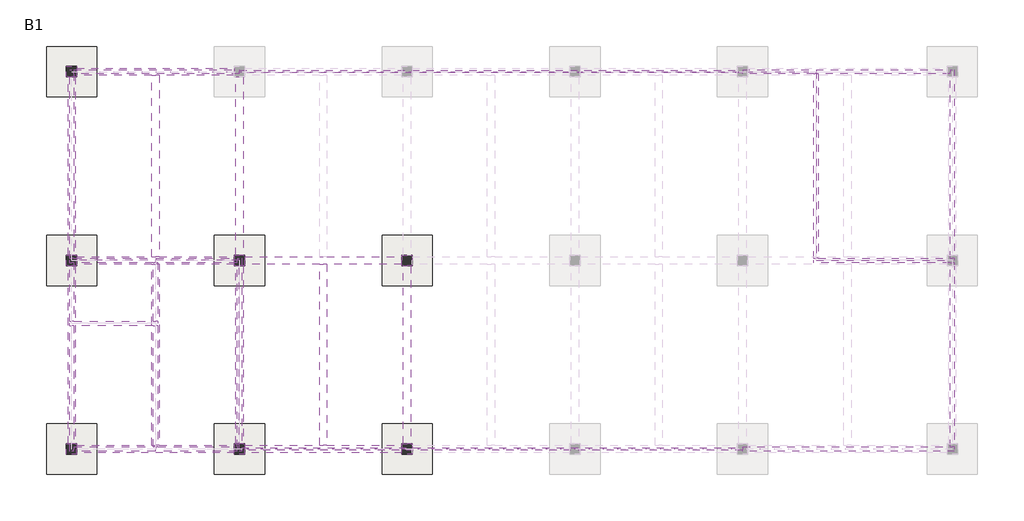
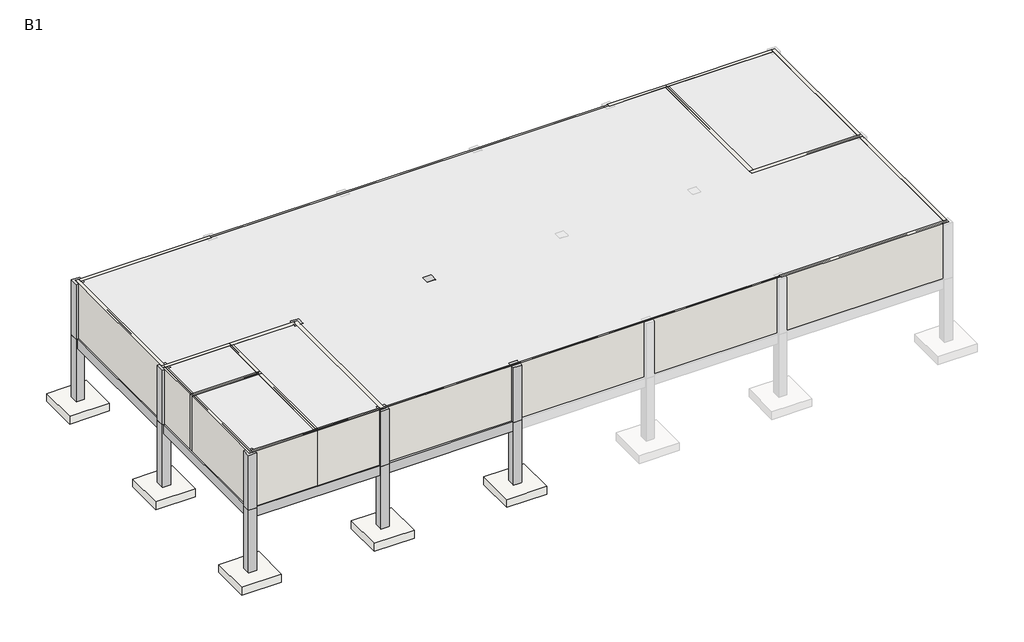
# One storey, part 1 of 2: 21 walls, 14 columns, 13 beams, 12 slabs.
"""IFC4 building model written with IfcOpenShell, lengths in millimetres."""

import ifcopenshell
import ifcopenshell.guid

model = None  # the IFC model being written
_history = None  # IfcOwnerHistory: only IFC2X3 demands one
_inside = {}  # id of a spatial element -> (the spatial element, [elements in it])
_under = {}  # id of a project, library or spatial element -> (it, [spatial elements below it])
_declared = {}  # id of a project -> (the project, [libraries it declares])
_typed = {}  # id of a type object -> (the type object, [elements of that type])
_made_of = {}  # id of a material, layer set ... -> (it, [elements and type objects made of it])


def new_model(schema):
    """Start an empty IFC model of exactly this schema.

    Asked for "IFC4X3", IfcOpenShell would pick the latest addendum, in which some entities
    have other attributes; the version numbers below select the first issue.
    IFC2X3 requires an IfcOwnerHistory on every rooted entity: one is made here for all.
    """
    global model, _history
    if schema == "IFC4X3":
        model = ifcopenshell.file(schema_version=(4, 3, 0, 0))
    else:
        model = ifcopenshell.file(schema=schema)
    _inside.clear()
    _under.clear()
    _declared.clear()
    _typed.clear()
    _made_of.clear()
    _history = None
    if model.schema == "IFC2X3":
        org = make("IfcOrganization", Name="unknown")
        user = make(
            "IfcPersonAndOrganization",
            ThePerson=make("IfcPerson", FamilyName="unknown"),
            TheOrganization=org,
        )
        app = make(
            "IfcApplication",
            ApplicationDeveloper=org,
            Version="unknown",
            ApplicationFullName="unknown",
            ApplicationIdentifier="unknown",
        )
        _history = make(
            "IfcOwnerHistory",
            OwningUser=user,
            OwningApplication=app,
            ChangeAction="ADDED",
            CreationDate=0,
        )
    return model


def make(cls, **values):
    """One entity of the class cls with the attributes given. An attribute that is None is left unset."""
    return model.create_entity(
        cls, **{name: value for name, value in values.items() if value is not None}
    )


def rooted(cls, **values):
    """An entity with a GlobalId (a new one), such as an element, a storey or a relation."""
    return make(cls, GlobalId=ifcopenshell.guid.new(), OwnerHistory=_history, **values)


def si_unit(unit_type, name, prefix=None):
    """IfcSIUnit, for example si_unit("LENGTHUNIT", "METRE", prefix="MILLI")."""
    return make("IfcSIUnit", UnitType=unit_type, Prefix=prefix, Name=name)


def assignment(units):
    """IfcUnitAssignment: the units of a project."""
    return None if units is None else make("IfcUnitAssignment", Units=units)


def point(xyz):
    """IfcCartesianPoint."""
    return None if xyz is None else make("IfcCartesianPoint", Coordinates=xyz)


def direction(xyz):
    """IfcDirection."""
    return None if xyz is None else make("IfcDirection", DirectionRatios=xyz)


def frame(location, z_axis=None, x_axis=None):
    """IfcAxis2Placement3D, a coordinate frame: its origin and axes. An axis left out is left unset."""
    return make(
        "IfcAxis2Placement3D",
        Location=point(location),
        Axis=direction(z_axis),
        RefDirection=direction(x_axis),
    )


def origin():
    """The frame at (0, 0, 0) with its axes left unset."""
    return frame((0.0, 0.0, 0.0))


def origin_with_axes():
    """The frame at (0, 0, 0) with the z axis (0, 0, 1) and the x axis (1, 0, 0) written out."""
    return frame((0.0, 0.0, 0.0), z_axis=(0.0, 0.0, 1.0), x_axis=(1.0, 0.0, 0.0))


def place(relative_to, where):
    """IfcLocalPlacement: puts the frame where relative to a parent placement (None: the world)."""
    return make(
        "IfcLocalPlacement", PlacementRelTo=relative_to, RelativePlacement=where
    )


def context(
    kind, dimensions, precision=None, world=None, true_north=None, identifier=None
):
    """IfcGeometricRepresentationContext, for example the 3D "Model" context."""
    return make(
        "IfcGeometricRepresentationContext",
        ContextIdentifier=identifier,
        ContextType=kind,
        CoordinateSpaceDimension=dimensions,
        Precision=precision,
        WorldCoordinateSystem=world,
        TrueNorth=true_north,
    )


def project(units=None, contexts=None):
    """IfcProject with its units and contexts."""
    return rooted(
        "IfcProject",
        Name="project",
        RepresentationContexts=contexts,
        UnitsInContext=assignment(units),
    )


def spatial(cls, under=None, at=None, **own):
    """A site, building, storey or space (cls), placed at a placement, below another one or the project."""
    s = rooted(cls, ObjectPlacement=at, **own)
    if under is not None:
        _under.setdefault(under.id(), (under, []))[1].append(s)
    return s


def polyline(points):
    """IfcPolyline through the points."""
    return make("IfcPolyline", Points=[point(p) for p in points])


def outline(outer, holes=None, kind="AREA"):
    """IfcArbitraryClosedProfileDef: a profile drawn as a closed curve; with holes, ...WithVoids."""
    if holes is None:
        return make("IfcArbitraryClosedProfileDef", ProfileType=kind, OuterCurve=outer)
    return make(
        "IfcArbitraryProfileDefWithVoids",
        ProfileType=kind,
        OuterCurve=outer,
        InnerCurves=holes,
    )


def extrude(swept, where, along, depth):
    """IfcExtrudedAreaSolid: the profile swept, set in the frame where, extruded along a direction by depth."""
    return make(
        "IfcExtrudedAreaSolid",
        SweptArea=swept,
        Position=where,
        ExtrudedDirection=direction(along),
        Depth=depth,
    )


def faces_of(points, faces, orient=None, outer=None):
    """IfcFace entities. A face is a list of loops; a loop is a list of indices into points, from 0.

    orient and outer hold one flag for each loop. By default every Orientation is true, the
    first loop of a face is its IfcFaceOuterBound and the others are IfcFaceBound.
    """
    made = []
    for i, loops in enumerate(faces):
        bounds = []
        for j, loop in enumerate(loops):
            is_outer = j == 0 if outer is None else outer[i][j]
            bounds.append(
                make(
                    "IfcFaceOuterBound" if is_outer else "IfcFaceBound",
                    Bound=make("IfcPolyLoop", Polygon=[points[k] for k in loop]),
                    Orientation=True if orient is None else orient[i][j],
                )
            )
        made.append(make("IfcFace", Bounds=bounds))
    return made


def faceted_brep(points, faces, orient=None, outer=None, voids=None):
    """IfcFacetedBrep: a solid bounded by flat faces; with voids (closed shells), ...WithVoids."""
    shared = [point(p) for p in points]
    hull = make("IfcClosedShell", CfsFaces=faces_of(shared, faces, orient, outer))
    if voids is None:
        return make("IfcFacetedBrep", Outer=hull)
    return make(
        "IfcFacetedBrepWithVoids",
        Outer=hull,
        Voids=[
            make(cls, CfsFaces=faces_of(shared, fs, o, b)) for cls, fs, o, b in voids
        ],
    )


def shape(context_of_items, identifier, shape_type, items):
    """IfcShapeRepresentation: the items that make up one representation, for example the "Body"."""
    return make(
        "IfcShapeRepresentation",
        ContextOfItems=context_of_items,
        RepresentationIdentifier=identifier,
        RepresentationType=shape_type,
        Items=items,
    )


def source(mapping_origin, context_of_items, identifier, shape_type, items):
    """IfcRepresentationMap: a shape defined once, which mapped items show again and again."""
    return make(
        "IfcRepresentationMap",
        MappingOrigin=mapping_origin,
        MappedRepresentation=shape(context_of_items, identifier, shape_type, items),
    )


def transform(
    local_origin,
    x_axis=None,
    y_axis=None,
    z_axis=None,
    scale=None,
    scale2=None,
    scale3=None,
    uniform=True,
):
    """IfcCartesianTransformationOperator3D, or its non-uniform kind. x_axis, y_axis, z_axis: its Axis1, 2, 3."""
    if uniform:
        return make(
            "IfcCartesianTransformationOperator3D",
            Axis1=direction(x_axis),
            Axis2=direction(y_axis),
            LocalOrigin=point(local_origin),
            Scale=scale,
            Axis3=direction(z_axis),
        )
    return make(
        "IfcCartesianTransformationOperator3DnonUniform",
        Axis1=direction(x_axis),
        Axis2=direction(y_axis),
        LocalOrigin=point(local_origin),
        Scale=scale,
        Axis3=direction(z_axis),
        Scale2=scale2,
        Scale3=scale3,
    )


def mapped(mapping_source, mapping_target):
    """IfcMappedItem: shows the shape of a source again, moved by a transform."""
    return make(
        "IfcMappedItem", MappingSource=mapping_source, MappingTarget=mapping_target
    )


def made_of(thing, what):
    """Note that an element or type object is made of a material, layer set ...; save() writes the relation."""
    if what is not None:
        _made_of.setdefault(what.id(), (what, []))[1].append(thing)
    return thing


def element(
    cls,
    number,
    at=None,
    inside=None,
    cuts=None,
    type_object=None,
    material=None,
    context=None,
    identifier="Body",
    shape_type=None,
    held_by="IfcProductDefinitionShape",
    body=None,
    shapes=None,
    **own,
):
    """One element of the class cls, such as IfcWall. Its Tag is "e" and its number.

    at: its placement. inside: the storey or other place that contains it. cuts: it is an
    opening in that element (IfcRelVoidsElement). A single representation is given by context,
    identifier, shape_type and body (its items); several are given by shapes. held_by: the class
    of the entity that holds the representations. save() writes the other relations.
    """
    e = rooted(cls, Tag="e%d" % number, ObjectPlacement=at, **own)
    if body is not None:
        shapes = [shape(context, identifier, shape_type, body)]
    if shapes is not None:
        e.Representation = make(held_by, Representations=shapes)
    if inside is not None:
        _inside.setdefault(inside.id(), (inside, []))[1].append(e)
    if cuts is not None:
        rooted(
            "IfcRelVoidsElement", RelatingBuildingElement=cuts, RelatedOpeningElement=e
        )
    if type_object is not None:
        _typed.setdefault(type_object.id(), (type_object, []))[1].append(e)
    return made_of(e, material)


def aggregate(whole, parts):
    """IfcRelAggregates: a whole, such as a stair, and the parts it consists of."""
    return rooted("IfcRelAggregates", RelatingObject=whole, RelatedObjects=parts)


def save(model, path):
    """Write the relations noted so far, then the file.

    IfcRelAggregates (storeys below a building ...), IfcRelContainedInSpatialStructure (elements
    in a storey), IfcRelDefinesByType, IfcRelAssociatesMaterial and IfcRelDeclares: one each for
    every whole, place, type object, material and project.
    """
    for whole, parts in _under.values():
        aggregate(whole, parts)
    for where, things in _inside.values():
        rooted(
            "IfcRelContainedInSpatialStructure",
            RelatedElements=things,
            RelatingStructure=where,
        )
    for kind, things in _typed.values():
        rooted("IfcRelDefinesByType", RelatedObjects=things, RelatingType=kind)
    for what, things in _made_of.values():
        rooted("IfcRelAssociatesMaterial", RelatedObjects=things, RelatingMaterial=what)
    for by, libraries in _declared.values():
        rooted("IfcRelDeclares", RelatingContext=by, RelatedDefinitions=libraries)
    model.write(path)


def ft112_footing_rectangular_ft112_2400x2400x500_5fe39465(model_context):
    return source(origin(), model_context, "Body", "SweptSolid", [
        extrude(outline(polyline([(1200.0, 1200.0), (1200.0, -1200.0), (-1200.0, -1200.0), (-1200.0, 1200.0), (1200.0, 1200.0)])), frame((0.0, 0.0, -500.0), z_axis=(0.0, 0.0, 1.0), x_axis=(1.0, 0.0, 0.0)), (0.0, 0.0, 1.0), 500.0),
    ])


model = new_model("IFC4")

# Units and contexts
model_context = context("Model", 3, world=origin())
ifc_project = project(units=[si_unit("LENGTHUNIT", "METRE", prefix="MILLI")], contexts=[model_context])

# Site, building, storey
site = spatial("IfcSite", under=ifc_project)
building = spatial("IfcBuilding", under=site)
storey = spatial("IfcBuildingStorey", under=building, Name="B1", Elevation=-4000.0)

# Beams
placement = place(None, origin())
element("IfcBeam", 1, ObjectType="Concrete-Rectangular-Beam : BM111_400x500_RG1", at=placement, inside=storey, context=model_context, shape_type="SweptSolid", body=[
    extrude(outline(polyline([(49284.6521483, 181748.8614395), (49634.6521483, 181748.8614395), (49634.6521483, 173098.8614395), (49284.6521483, 173098.8614395), (49284.6521483, 181748.8614395)])), frame((0.0, 0.0, -600.0), z_axis=(0.0, 0.0, 1.0), x_axis=(1.0, 0.0, 0.0)), (0.0, 0.0, 1.0), 600.0),
])
element("IfcBeam", 2, ObjectType="Concrete-Rectangular-Beam : BM111_400x500_RG1", at=placement, inside=storey, context=model_context, shape_type="SweptSolid", body=[
    extrude(outline(polyline([(49284.6521483, 172748.8614395), (49634.6521483, 172748.8614395), (49634.6521483, 164098.8614395), (49284.6521483, 164098.8614395), (49284.6521483, 172748.8614395)])), frame((0.0, 0.0, -600.0), z_axis=(0.0, 0.0, 1.0), x_axis=(1.0, 0.0, 0.0)), (0.0, 0.0, 1.0), 600.0),
])
element("IfcBeam", 3, ObjectType="Concrete-Rectangular-Beam : BM111_400x500_RG1", at=placement, inside=storey, context=model_context, shape_type="SweptSolid", body=[
    extrude(outline(polyline([(57284.6521483, 172748.8614395), (57634.6521483, 172748.8614395), (57634.6521483, 164098.8614395), (57284.6521483, 164098.8614395), (57284.6521483, 172748.8614395)])), frame((0.0, 0.0, -600.0), z_axis=(0.0, 0.0, 1.0), x_axis=(1.0, 0.0, 0.0)), (0.0, 0.0, 1.0), 600.0),
])
element("IfcBeam", 4, ObjectType="Concrete-Rectangular-Beam : BM111_400x500_RG1", at=placement, inside=storey, context=model_context, shape_type="Brep", body=[
    faceted_brep([(45709.6521483, 182098.8614395, 0.0), (45709.6521483, 181748.8614395, 0.0), (49284.6521483, 181748.8614395, 0.0), (49634.6521483, 181748.8614395, 0.0), (53209.6521483, 181748.8614395, 0.0), (53209.6521483, 182098.8614395, 0.0), (45709.6521483, 181748.8614395, -600.0), (49284.6521483, 181748.8614395, -600.0), (49634.6521483, 181748.8614395, -600.0), (53209.6521483, 181748.8614395, -600.0), (45709.6521483, 182098.8614395, -600.0), (53209.6521483, 182098.8614395, -600.0)], [[[0, 1, 2, 3, 4, 5]], [[1, 6, 7, 8, 9, 4, 3, 2]], [[6, 10, 11, 9, 8, 7]], [[10, 0, 5, 11]], [[1, 0, 10, 6]], [[5, 4, 9, 11]]]),
])
element("IfcBeam", 5, ObjectType="Concrete-Rectangular-Beam : BM111_400x500_RG1", at=placement, inside=storey, context=model_context, shape_type="Brep", body=[
    faceted_brep([(45709.6521483, 173098.8614395, 0.0), (45709.6521483, 172748.8614395, 0.0), (49284.6521483, 172748.8614395, 0.0), (49634.6521483, 172748.8614395, 0.0), (53209.6521483, 172748.8614395, 0.0), (53209.6521483, 173098.8614395, 0.0), (49634.6521483, 173098.8614395, 0.0), (49284.6521483, 173098.8614395, 0.0), (45709.6521483, 172748.8614395, -600.0), (49284.6521483, 172748.8614395, -600.0), (49634.6521483, 172748.8614395, -600.0), (53209.6521483, 172748.8614395, -600.0), (45709.6521483, 173098.8614395, -600.0), (49284.6521483, 173098.8614395, -600.0), (49634.6521483, 173098.8614395, -600.0), (53209.6521483, 173098.8614395, -600.0)], [[[0, 1, 2, 3, 4, 5, 6, 7]], [[1, 8, 9, 10, 11, 4, 3, 2]], [[8, 12, 13, 14, 15, 11, 10, 9]], [[12, 0, 7, 6, 5, 15, 14, 13]], [[1, 0, 12, 8]], [[5, 4, 11, 15]]]),
])
element("IfcBeam", 6, ObjectType="Concrete-Rectangular-Beam : BM111_400x500_RG1", at=placement, inside=storey, context=model_context, shape_type="Brep", body=[
    faceted_brep([(53709.6521483, 173098.8614395, 0.0), (53709.6521483, 172748.8614395, 0.0), (57284.6521483, 172748.8614395, 0.0), (57634.6521483, 172748.8614395, 0.0), (61209.6521483, 172748.8614395, 0.0), (61209.6521483, 173098.8614395, 0.0), (57634.6521483, 173098.8614395, 0.0), (57284.6521483, 173098.8614395, 0.0), (53709.6521483, 172748.8614395, -600.0), (57284.6521483, 172748.8614395, -600.0), (57634.6521483, 172748.8614395, -600.0), (61209.6521483, 172748.8614395, -600.0), (53709.6521483, 173098.8614395, -600.0), (57284.6521483, 173098.8614395, -600.0), (57634.6521483, 173098.8614395, -600.0), (61209.6521483, 173098.8614395, -600.0)], [[[0, 1, 2, 3, 4, 5, 6, 7]], [[1, 8, 9, 10, 11, 4, 3, 2]], [[8, 12, 13, 14, 15, 11, 10, 9]], [[12, 0, 7, 6, 5, 15, 14, 13]], [[1, 0, 12, 8]], [[5, 4, 11, 15]]]),
])
element("IfcBeam", 7, ObjectType="Concrete-Rectangular-Beam : BM111_400x500_RG1", at=placement, inside=storey, context=model_context, shape_type="Brep", body=[
    faceted_brep([(45709.6521483, 164098.8614395, 0.0), (45709.6521483, 163748.8614395, 0.0), (53209.6521483, 163748.8614395, 0.0), (53209.6521483, 164098.8614395, 0.0), (49634.6521483, 164098.8614395, 0.0), (49284.6521483, 164098.8614395, 0.0), (45709.6521483, 163748.8614395, -600.0), (53209.6521483, 163748.8614395, -600.0), (45709.6521483, 164098.8614395, -600.0), (49284.6521483, 164098.8614395, -600.0), (49634.6521483, 164098.8614395, -600.0), (53209.6521483, 164098.8614395, -600.0)], [[[0, 1, 2, 3, 4, 5]], [[1, 6, 7, 2]], [[6, 8, 9, 10, 11, 7]], [[8, 0, 5, 4, 3, 11, 10, 9]], [[1, 0, 8, 6]], [[3, 2, 7, 11]]]),
])
element("IfcBeam", 8, ObjectType="Concrete-Rectangular-Beam : BM111_400x500_RG1", at=placement, inside=storey, context=model_context, shape_type="Brep", body=[
    faceted_brep([(53709.6521483, 164098.8614395, 0.0), (53709.6521483, 163748.8614395, 0.0), (61209.6521483, 163748.8614395, 0.0), (61209.6521483, 164098.8614395, 0.0), (57634.6521483, 164098.8614395, 0.0), (57284.6521483, 164098.8614395, 0.0), (53709.6521483, 163748.8614395, -600.0), (61209.6521483, 163748.8614395, -600.0), (53709.6521483, 164098.8614395, -600.0), (57284.6521483, 164098.8614395, -600.0), (57634.6521483, 164098.8614395, -600.0), (61209.6521483, 164098.8614395, -600.0)], [[[0, 1, 2, 3, 4, 5]], [[1, 6, 7, 2]], [[6, 8, 9, 10, 11, 7]], [[8, 0, 5, 4, 3, 11, 10, 9]], [[1, 0, 8, 6]], [[3, 2, 7, 11]]]),
])
element("IfcBeam", 9, ObjectType="Concrete-Rectangular-Beam : BM111_400x500_RG1", at=placement, inside=storey, context=model_context, shape_type="SweptSolid", body=[
    extrude(outline(polyline([(45284.6521483, 181673.8614395), (45634.6521483, 181673.8614395), (45634.6521483, 173173.8614395), (45284.6521483, 173173.8614395), (45284.6521483, 181673.8614395)])), frame((0.0, 0.0, -600.0), z_axis=(0.0, 0.0, 1.0), x_axis=(1.0, 0.0, 0.0)), (0.0, 0.0, 1.0), 600.0),
])
element("IfcBeam", 10, ObjectType="Concrete-Rectangular-Beam : BM111_400x500_RG1", at=placement, inside=storey, context=model_context, shape_type="SweptSolid", body=[
    extrude(outline(polyline([(45284.6521483, 172673.8614395), (45634.6521483, 172673.8614395), (45634.6521483, 164173.8614395), (45284.6521483, 164173.8614395), (45284.6521483, 172673.8614395)])), frame((0.0, 0.0, -600.0), z_axis=(0.0, 0.0, 1.0), x_axis=(1.0, 0.0, 0.0)), (0.0, 0.0, 1.0), 600.0),
])
element("IfcBeam", 11, ObjectType="Concrete-Rectangular-Beam : BM111_400x500_RG1", at=placement, inside=storey, context=model_context, shape_type="SweptSolid", body=[
    extrude(outline(polyline([(53284.6521483, 181673.8614395), (53634.6521483, 181673.8614395), (53634.6521483, 173173.8614395), (53284.6521483, 173173.8614395), (53284.6521483, 181673.8614395)])), frame((0.0, 0.0, -600.0), z_axis=(0.0, 0.0, 1.0), x_axis=(1.0, 0.0, 0.0)), (0.0, 0.0, 1.0), 600.0),
])
element("IfcBeam", 12, ObjectType="Concrete-Rectangular-Beam : BM111_400x500_RG1", at=placement, inside=storey, context=model_context, shape_type="SweptSolid", body=[
    extrude(outline(polyline([(53284.6521483, 172673.8614395), (53634.6521483, 172673.8614395), (53634.6521483, 164173.8614395), (53284.6521483, 164173.8614395), (53284.6521483, 172673.8614395)])), frame((0.0, 0.0, -600.0), z_axis=(0.0, 0.0, 1.0), x_axis=(1.0, 0.0, 0.0)), (0.0, 0.0, 1.0), 600.0),
])
element("IfcBeam", 13, ObjectType="Concrete-Rectangular-Beam : BM111_400x500_RG1", at=placement, inside=storey, context=model_context, shape_type="SweptSolid", body=[
    extrude(outline(polyline([(61284.6521483, 172673.8614395), (61634.6521483, 172673.8614395), (61634.6521483, 164173.8614395), (61284.6521483, 164173.8614395), (61284.6521483, 172673.8614395)])), frame((0.0, 0.0, -600.0), z_axis=(0.0, 0.0, 1.0), x_axis=(1.0, 0.0, 0.0)), (0.0, 0.0, 1.0), 600.0),
])

# Columns
element("IfcColumn", 14, ObjectType="Concrete-Rectangular-Column : CL111_500x500", at=placement, inside=storey, context=model_context, shape_type="Brep", body=[
    faceted_brep([(45709.6521483, 182173.8614395, 0.0), (45709.6521483, 181673.8614395, 0.0), (45209.6521483, 181673.8614395, 0.0), (45209.6521483, 182173.8614395, 0.0), (45709.6521483, 182173.8614395, 3500.0), (45709.6521483, 182098.8614395, 3500.0), (45709.6521483, 181748.8614395, 3500.0), (45709.6521483, 181673.8614395, 3500.0), (45634.6521483, 181673.8614395, 3500.0), (45284.6521483, 181673.8614395, 3500.0), (45209.6521483, 181673.8614395, 3500.0), (45209.6521483, 182173.8614395, 3500.0)], [[[0, 1, 2, 3]], [[4, 5, 6, 7, 1, 0]], [[7, 8, 9, 10, 2, 1]], [[10, 11, 3, 2]], [[11, 4, 0, 3]], [[4, 11, 10, 9, 8, 7, 6, 5]]]),
])
element("IfcColumn", 15, ObjectType="Concrete-Rectangular-Column : CL111_500x500", at=placement, inside=storey, context=model_context, shape_type="Brep", body=[
    faceted_brep([(45709.6521483, 173173.8614395, 0.0), (45709.6521483, 172673.8614395, 0.0), (45209.6521483, 172673.8614395, 0.0), (45209.6521483, 173173.8614395, 0.0), (45709.6521483, 173173.8614395, 3500.0), (45709.6521483, 173098.8614395, 3500.0), (45709.6521483, 172748.8614395, 3500.0), (45709.6521483, 172673.8614395, 3500.0), (45634.6521483, 172673.8614395, 3500.0), (45284.6521483, 172673.8614395, 3500.0), (45209.6521483, 172673.8614395, 3500.0), (45209.6521483, 173173.8614395, 3500.0), (45284.6521483, 173173.8614395, 3500.0), (45634.6521483, 173173.8614395, 3500.0)], [[[0, 1, 2, 3]], [[4, 5, 6, 7, 1, 0]], [[7, 8, 9, 10, 2, 1]], [[10, 11, 3, 2]], [[11, 12, 13, 4, 0, 3]], [[4, 13, 12, 11, 10, 9, 8, 7, 6, 5]]]),
])
element("IfcColumn", 16, ObjectType="Concrete-Rectangular-Column : CL111_500x500", at=placement, inside=storey, context=model_context, shape_type="Brep", body=[
    faceted_brep([(53709.6521483, 173173.8614395, 0.0), (53709.6521483, 172673.8614395, 0.0), (53209.6521483, 172673.8614395, 0.0), (53209.6521483, 173173.8614395, 0.0), (53709.6521483, 173173.8614395, 3500.0), (53709.6521483, 173098.8614395, 3500.0), (53709.6521483, 172748.8614395, 3500.0), (53709.6521483, 172673.8614395, 3500.0), (53634.6521483, 172673.8614395, 3500.0), (53284.6521483, 172673.8614395, 3500.0), (53209.6521483, 172673.8614395, 3500.0), (53209.6521483, 172748.8614395, 3500.0), (53209.6521483, 173098.8614395, 3500.0), (53209.6521483, 173173.8614395, 3500.0), (53284.6521483, 173173.8614395, 3500.0), (53634.6521483, 173173.8614395, 3500.0)], [[[0, 1, 2, 3]], [[4, 5, 6, 7, 1, 0]], [[7, 8, 9, 10, 2, 1]], [[10, 11, 12, 13, 3, 2]], [[13, 14, 15, 4, 0, 3]], [[4, 15, 14, 13, 12, 11, 10, 9, 8, 7, 6, 5]]]),
])
element("IfcColumn", 17, ObjectType="Concrete-Rectangular-Column : CL111_500x500", at=placement, inside=storey, context=model_context, shape_type="Brep", body=[
    faceted_brep([(61709.6521483, 173173.8614395, 0.0), (61709.6521483, 172673.8614395, 0.0), (61209.6521483, 172673.8614395, 0.0), (61209.6521483, 173173.8614395, 0.0), (61709.6521483, 173173.8614395, 3500.0), (61709.6521483, 173098.8614395, 3500.0), (61709.6521483, 172748.8614395, 3500.0), (61709.6521483, 172673.8614395, 3500.0), (61634.6521483, 172673.8614395, 3500.0), (61284.6521483, 172673.8614395, 3500.0), (61209.6521483, 172673.8614395, 3500.0), (61209.6521483, 172748.8614395, 3500.0), (61209.6521483, 173098.8614395, 3500.0), (61209.6521483, 173173.8614395, 3500.0), (61284.6521483, 173173.8614395, 3500.0), (61634.6521483, 173173.8614395, 3500.0)], [[[0, 1, 2, 3]], [[4, 5, 6, 7, 1, 0]], [[7, 8, 9, 10, 2, 1]], [[10, 11, 12, 13, 3, 2]], [[13, 14, 15, 4, 0, 3]], [[4, 15, 14, 13, 12, 11, 10, 9, 8, 7, 6, 5]]]),
])
element("IfcColumn", 18, ObjectType="Concrete-Rectangular-Column : CL111_500x500", at=placement, inside=storey, context=model_context, shape_type="Brep", body=[
    faceted_brep([(45709.6521483, 164173.8614395, 0.0), (45709.6521483, 163673.8614395, 0.0), (45209.6521483, 163673.8614395, 0.0), (45209.6521483, 164173.8614395, 0.0), (45709.6521483, 164173.8614395, 3500.0), (45709.6521483, 164098.8614395, 3500.0), (45709.6521483, 163748.8614395, 3500.0), (45709.6521483, 163673.8614395, 3500.0), (45209.6521483, 163673.8614395, 3500.0), (45209.6521483, 164173.8614395, 3500.0), (45284.6521483, 164173.8614395, 3500.0), (45634.6521483, 164173.8614395, 3500.0)], [[[0, 1, 2, 3]], [[4, 5, 6, 7, 1, 0]], [[7, 8, 2, 1]], [[8, 9, 3, 2]], [[9, 10, 11, 4, 0, 3]], [[4, 11, 10, 9, 8, 7, 6, 5]]]),
])
element("IfcColumn", 19, ObjectType="Concrete-Rectangular-Column : CL111_500x500", at=placement, inside=storey, context=model_context, shape_type="Brep", body=[
    faceted_brep([(53709.6521483, 164173.8614395, 0.0), (53709.6521483, 163673.8614395, 0.0), (53209.6521483, 163673.8614395, 0.0), (53209.6521483, 164173.8614395, 0.0), (53709.6521483, 164173.8614395, 3500.0), (53709.6521483, 164098.8614395, 3500.0), (53709.6521483, 163748.8614395, 3500.0), (53709.6521483, 163673.8614395, 3500.0), (53209.6521483, 163673.8614395, 3500.0), (53209.6521483, 163748.8614395, 3500.0), (53209.6521483, 164098.8614395, 3500.0), (53209.6521483, 164173.8614395, 3500.0), (53284.6521483, 164173.8614395, 3500.0), (53634.6521483, 164173.8614395, 3500.0)], [[[0, 1, 2, 3]], [[4, 5, 6, 7, 1, 0]], [[7, 8, 2, 1]], [[8, 9, 10, 11, 3, 2]], [[11, 12, 13, 4, 0, 3]], [[4, 13, 12, 11, 10, 9, 8, 7, 6, 5]]]),
])
element("IfcColumn", 20, ObjectType="Concrete-Rectangular-Column : CL111_500x500", at=placement, inside=storey, context=model_context, shape_type="Brep", body=[
    faceted_brep([(61709.6521483, 164173.8614395, 0.0), (61709.6521483, 163673.8614395, 0.0), (61209.6521483, 163673.8614395, 0.0), (61209.6521483, 164173.8614395, 0.0), (61709.6521483, 164173.8614395, 3500.0), (61709.6521483, 164098.8614395, 3500.0), (61709.6521483, 163748.8614395, 3500.0), (61709.6521483, 163673.8614395, 3500.0), (61209.6521483, 163673.8614395, 3500.0), (61209.6521483, 163748.8614395, 3500.0), (61209.6521483, 164098.8614395, 3500.0), (61209.6521483, 164173.8614395, 3500.0), (61284.6521483, 164173.8614395, 3500.0), (61634.6521483, 164173.8614395, 3500.0)], [[[0, 1, 2, 3]], [[4, 5, 6, 7, 1, 0]], [[7, 8, 2, 1]], [[8, 9, 10, 11, 3, 2]], [[11, 12, 13, 4, 0, 3]], [[4, 13, 12, 11, 10, 9, 8, 7, 6, 5]]]),
])
element("IfcColumn", 21, ObjectType="Concrete-Rectangular-Column : CL111_500x500", at=placement, inside=storey, context=model_context, shape_type="Brep", body=[
    faceted_brep([(45709.6521483, 182173.8614395, -4000.0), (45709.6521483, 181673.8614395, -4000.0), (45209.6521483, 181673.8614395, -4000.0), (45209.6521483, 182173.8614395, -4000.0), (45709.6521483, 182173.8614395, 0.0), (45709.6521483, 182098.8614395, 0.0), (45709.6521483, 181748.8614395, 0.0), (45709.6521483, 181673.8614395, 0.0), (45634.6521483, 181673.8614395, 0.0), (45284.6521483, 181673.8614395, 0.0), (45209.6521483, 181673.8614395, 0.0), (45209.6521483, 182173.8614395, 0.0)], [[[0, 1, 2, 3]], [[4, 5, 6, 7, 1, 0]], [[7, 8, 9, 10, 2, 1]], [[10, 11, 3, 2]], [[11, 4, 0, 3]], [[4, 11, 10, 9, 8, 7, 6, 5]]]),
])
element("IfcColumn", 22, ObjectType="Concrete-Rectangular-Column : CL111_500x500", at=placement, inside=storey, context=model_context, shape_type="Brep", body=[
    faceted_brep([(45709.6521483, 173173.8614395, -4000.0), (45709.6521483, 172673.8614395, -4000.0), (45209.6521483, 172673.8614395, -4000.0), (45209.6521483, 173173.8614395, -4000.0), (45709.6521483, 173173.8614395, 0.0), (45709.6521483, 173098.8614395, 0.0), (45709.6521483, 172748.8614395, 0.0), (45709.6521483, 172673.8614395, 0.0), (45634.6521483, 172673.8614395, 0.0), (45284.6521483, 172673.8614395, 0.0), (45209.6521483, 172673.8614395, 0.0), (45209.6521483, 173173.8614395, 0.0), (45284.6521483, 173173.8614395, 0.0), (45634.6521483, 173173.8614395, 0.0)], [[[0, 1, 2, 3]], [[4, 5, 6, 7, 1, 0]], [[7, 8, 9, 10, 2, 1]], [[10, 11, 3, 2]], [[11, 12, 13, 4, 0, 3]], [[4, 13, 12, 11, 10, 9, 8, 7, 6, 5]]]),
])
element("IfcColumn", 23, ObjectType="Concrete-Rectangular-Column : CL111_500x500", at=placement, inside=storey, context=model_context, shape_type="Brep", body=[
    faceted_brep([(53709.6521483, 173173.8614395, -4000.0), (53709.6521483, 172673.8614395, -4000.0), (53209.6521483, 172673.8614395, -4000.0), (53209.6521483, 173173.8614395, -4000.0), (53709.6521483, 173173.8614395, 0.0), (53709.6521483, 173098.8614395, 0.0), (53709.6521483, 172748.8614395, 0.0), (53709.6521483, 172673.8614395, 0.0), (53634.6521483, 172673.8614395, 0.0), (53284.6521483, 172673.8614395, 0.0), (53209.6521483, 172673.8614395, 0.0), (53209.6521483, 172748.8614395, 0.0), (53209.6521483, 173098.8614395, 0.0), (53209.6521483, 173173.8614395, 0.0), (53284.6521483, 173173.8614395, 0.0), (53634.6521483, 173173.8614395, 0.0)], [[[0, 1, 2, 3]], [[4, 5, 6, 7, 1, 0]], [[7, 8, 9, 10, 2, 1]], [[10, 11, 12, 13, 3, 2]], [[13, 14, 15, 4, 0, 3]], [[4, 15, 14, 13, 12, 11, 10, 9, 8, 7, 6, 5]]]),
])
element("IfcColumn", 24, ObjectType="Concrete-Rectangular-Column : CL111_500x500", at=placement, inside=storey, context=model_context, shape_type="Brep", body=[
    faceted_brep([(61709.6521483, 173173.8614395, -4000.0), (61709.6521483, 172673.8614395, -4000.0), (61209.6521483, 172673.8614395, -4000.0), (61209.6521483, 173173.8614395, -4000.0), (61709.6521483, 173173.8614395, 0.0), (61709.6521483, 173098.8614395, 0.0), (61709.6521483, 172748.8614395, 0.0), (61709.6521483, 172673.8614395, 0.0), (61634.6521483, 172673.8614395, 0.0), (61284.6521483, 172673.8614395, 0.0), (61209.6521483, 172673.8614395, 0.0), (61209.6521483, 172748.8614395, 0.0), (61209.6521483, 173098.8614395, 0.0), (61209.6521483, 173173.8614395, 0.0), (61284.6521483, 173173.8614395, 0.0), (61634.6521483, 173173.8614395, 0.0)], [[[0, 1, 2, 3]], [[4, 5, 6, 7, 1, 0]], [[7, 8, 9, 10, 2, 1]], [[10, 11, 12, 13, 3, 2]], [[13, 14, 15, 4, 0, 3]], [[4, 15, 14, 13, 12, 11, 10, 9, 8, 7, 6, 5]]]),
])
element("IfcColumn", 25, ObjectType="Concrete-Rectangular-Column : CL111_500x500", at=placement, inside=storey, context=model_context, shape_type="Brep", body=[
    faceted_brep([(45709.6521483, 164173.8614395, -4000.0), (45709.6521483, 163673.8614395, -4000.0), (45209.6521483, 163673.8614395, -4000.0), (45209.6521483, 164173.8614395, -4000.0), (45709.6521483, 164173.8614395, 0.0), (45709.6521483, 164098.8614395, 0.0), (45709.6521483, 163748.8614395, 0.0), (45709.6521483, 163673.8614395, 0.0), (45209.6521483, 163673.8614395, 0.0), (45209.6521483, 164173.8614395, 0.0), (45284.6521483, 164173.8614395, 0.0), (45634.6521483, 164173.8614395, 0.0)], [[[0, 1, 2, 3]], [[4, 5, 6, 7, 1, 0]], [[7, 8, 2, 1]], [[8, 9, 3, 2]], [[9, 10, 11, 4, 0, 3]], [[4, 11, 10, 9, 8, 7, 6, 5]]]),
])
element("IfcColumn", 26, ObjectType="Concrete-Rectangular-Column : CL111_500x500", at=placement, inside=storey, context=model_context, shape_type="Brep", body=[
    faceted_brep([(53709.6521483, 164173.8614395, -4000.0), (53709.6521483, 163673.8614395, -4000.0), (53209.6521483, 163673.8614395, -4000.0), (53209.6521483, 164173.8614395, -4000.0), (53709.6521483, 164173.8614395, 0.0), (53709.6521483, 164098.8614395, 0.0), (53709.6521483, 163748.8614395, 0.0), (53709.6521483, 163673.8614395, 0.0), (53209.6521483, 163673.8614395, 0.0), (53209.6521483, 163748.8614395, 0.0), (53209.6521483, 164098.8614395, 0.0), (53209.6521483, 164173.8614395, 0.0), (53284.6521483, 164173.8614395, 0.0), (53634.6521483, 164173.8614395, 0.0)], [[[0, 1, 2, 3]], [[4, 5, 6, 7, 1, 0]], [[7, 8, 2, 1]], [[8, 9, 10, 11, 3, 2]], [[11, 12, 13, 4, 0, 3]], [[4, 13, 12, 11, 10, 9, 8, 7, 6, 5]]]),
])
element("IfcColumn", 27, ObjectType="Concrete-Rectangular-Column : CL111_500x500", at=placement, inside=storey, context=model_context, shape_type="Brep", body=[
    faceted_brep([(61709.6521483, 164173.8614395, -4000.0), (61709.6521483, 163673.8614395, -4000.0), (61209.6521483, 163673.8614395, -4000.0), (61209.6521483, 164173.8614395, -4000.0), (61709.6521483, 164173.8614395, 0.0), (61709.6521483, 164098.8614395, 0.0), (61709.6521483, 163748.8614395, 0.0), (61709.6521483, 163673.8614395, 0.0), (61209.6521483, 163673.8614395, 0.0), (61209.6521483, 163748.8614395, 0.0), (61209.6521483, 164098.8614395, 0.0), (61209.6521483, 164173.8614395, 0.0), (61284.6521483, 164173.8614395, 0.0), (61634.6521483, 164173.8614395, 0.0)], [[[0, 1, 2, 3]], [[4, 5, 6, 7, 1, 0]], [[7, 8, 2, 1]], [[8, 9, 10, 11, 3, 2]], [[11, 12, 13, 4, 0, 3]], [[4, 13, 12, 11, 10, 9, 8, 7, 6, 5]]]),
])

# Slabs
element("IfcSlab", 28, ObjectType="CFS11_Slab RC_T150", at=placement, inside=storey, context=model_context, shape_type="SweptSolid", body=[
    extrude(outline(polyline([(87459.6521483, 181923.8614395), (87459.6521483, 172923.8614395), (80959.6521483, 172923.8614395), (80959.6521483, 181923.8614395), (87459.6521483, 181923.8614395)])), frame((0.0, 0.0, -150.0), z_axis=(0.0, 0.0, 1.0), x_axis=(1.0, 0.0, 0.0)), (0.0, 0.0, 1.0), 150.0),
])
element("IfcSlab", 29, ObjectType="CFS11_Slab RC_T150", at=placement, inside=storey, context=model_context, shape_type="SweptSolid", body=[
    extrude(outline(polyline([(53459.6521483, 163923.8614395), (49459.6521483, 163923.8614395), (49459.6521483, 172923.8614395), (53459.6521483, 172923.8614395), (53459.6521483, 163923.8614395)])), frame((0.0, 0.0, -150.0), z_axis=(0.0, 0.0, 1.0), x_axis=(1.0, 0.0, 0.0)), (0.0, 0.0, 1.0), 150.0),
])
element("IfcSlab", 30, ObjectType="CFS11_Slab RC_T150", at=placement, inside=storey, context=model_context, shape_type="SweptSolid", body=[
    extrude(outline(polyline([(80959.6521483, 181923.8614395), (80959.6521483, 172923.8614395), (87459.6521483, 172923.8614395), (87459.6521483, 163923.8614395), (53459.6521483, 163923.8614395), (53459.6521483, 172923.8614395), (45459.6521483, 172923.8614395), (45459.6521483, 181923.8614395), (80959.6521483, 181923.8614395)])), frame((0.0, 0.0, -150.0), z_axis=(0.0, 0.0, 1.0), x_axis=(1.0, 0.0, 0.0)), (0.0, 0.0, 1.0), 150.0),
])
element("IfcSlab", 31, ObjectType="CFS11_Slab RC_T150", at=placement, inside=storey, context=model_context, shape_type="SweptSolid", body=[
    extrude(outline(polyline([(45459.6521483, 163923.8614395), (45459.6521483, 169923.8614395), (49459.6521483, 169923.8614395), (49459.6521483, 163923.8614395), (45459.6521483, 163923.8614395)])), frame((0.0, 0.0, -150.0), z_axis=(0.0, 0.0, 1.0), x_axis=(1.0, 0.0, 0.0)), (0.0, 0.0, 1.0), 150.0),
])
element("IfcSlab", 32, ObjectType="CFS11_Slab RC_T150", at=placement, inside=storey, context=model_context, shape_type="SweptSolid", body=[
    extrude(outline(polyline([(45459.6521483, 172923.8614395), (49459.6521483, 172923.8614395), (49459.6521483, 169923.8614395), (45459.6521483, 169923.8614395), (45459.6521483, 172923.8614395)])), frame((0.0, 0.0, -150.0), z_axis=(0.0, 0.0, 1.0), x_axis=(1.0, 0.0, 0.0)), (0.0, 0.0, 1.0), 150.0),
])
ft112_footing_rectangular_ft112_2400x2400x500_shape = ft112_footing_rectangular_ft112_2400x2400x500_5fe39465(model_context)
element("IfcSlab", 33, ObjectType="FT112-Footing-Rectangular : FT112_2400x2400x500", at=placement, inside=storey, context=model_context, shape_type="MappedRepresentation", body=[
    mapped(ft112_footing_rectangular_ft112_2400x2400x500_shape, transform((45459.6521483, 181923.8614395, -4000.0), x_axis=(1.0, 0.0, 0.0), y_axis=(0.0, 1.0, 0.0), z_axis=(0.0, 0.0, 1.0))),
])
element("IfcSlab", 34, ObjectType="FT112-Footing-Rectangular : FT112_2400x2400x500", at=placement, inside=storey, context=model_context, shape_type="MappedRepresentation", body=[
    mapped(ft112_footing_rectangular_ft112_2400x2400x500_shape, transform((45459.6521483, 172923.8614395, -4000.0), x_axis=(1.0, 0.0, 0.0), y_axis=(0.0, 1.0, 0.0), z_axis=(0.0, 0.0, 1.0))),
])
element("IfcSlab", 35, ObjectType="FT112-Footing-Rectangular : FT112_2400x2400x500", at=placement, inside=storey, context=model_context, shape_type="MappedRepresentation", body=[
    mapped(ft112_footing_rectangular_ft112_2400x2400x500_shape, transform((53459.6521483, 172923.8614395, -4000.0), x_axis=(1.0, 0.0, 0.0), y_axis=(0.0, 1.0, 0.0), z_axis=(0.0, 0.0, 1.0))),
])
element("IfcSlab", 36, ObjectType="FT112-Footing-Rectangular : FT112_2400x2400x500", at=placement, inside=storey, context=model_context, shape_type="MappedRepresentation", body=[
    mapped(ft112_footing_rectangular_ft112_2400x2400x500_shape, transform((61459.6521483, 172923.8614395, -4000.0), x_axis=(1.0, 0.0, 0.0), y_axis=(0.0, 1.0, 0.0), z_axis=(0.0, 0.0, 1.0))),
])
element("IfcSlab", 37, ObjectType="FT112-Footing-Rectangular : FT112_2400x2400x500", at=placement, inside=storey, context=model_context, shape_type="MappedRepresentation", body=[
    mapped(ft112_footing_rectangular_ft112_2400x2400x500_shape, transform((45459.6521483, 163923.8614395, -4000.0), x_axis=(1.0, 0.0, 0.0), y_axis=(0.0, 1.0, 0.0), z_axis=(0.0, 0.0, 1.0))),
])
element("IfcSlab", 38, ObjectType="FT112-Footing-Rectangular : FT112_2400x2400x500", at=placement, inside=storey, context=model_context, shape_type="MappedRepresentation", body=[
    mapped(ft112_footing_rectangular_ft112_2400x2400x500_shape, transform((53459.6521483, 163923.8614395, -4000.0), x_axis=(1.0, 0.0, 0.0), y_axis=(0.0, 1.0, 0.0), z_axis=(0.0, 0.0, 1.0))),
])
element("IfcSlab", 39, ObjectType="FT112-Footing-Rectangular : FT112_2400x2400x500", at=placement, inside=storey, context=model_context, shape_type="MappedRepresentation", body=[
    mapped(ft112_footing_rectangular_ft112_2400x2400x500_shape, transform((61459.6521483, 163923.8614395, -4000.0), x_axis=(1.0, 0.0, 0.0), y_axis=(0.0, 1.0, 0.0), z_axis=(0.0, 0.0, 1.0))),
])

# Walls
element("IfcWall", 40, ObjectType="WA111-Exterior RC Wall 200mm", at=placement, inside=storey, context=model_context, shape_type="Brep", body=[
    faceted_brep([(80959.6521483, 181823.8614395, 0.0), (81066.6521483, 181823.8614395, 0.0), (87359.6521483, 181823.8614395, 0.0), (87359.6521483, 181823.8614395, 3500.0), (81066.6521483, 181823.8614395, 3500.0), (80959.6521483, 181823.8614395, 3500.0), (80959.6521483, 182023.8614395, 0.0), (80959.6521483, 182023.8614395, 3500.0), (87359.6521483, 182023.8614395, 3500.0), (87359.6521483, 182023.8614395, 0.0)], [[[0, 1, 2, 3, 4, 5]], [[6, 7, 8, 9]], [[2, 1, 0, 6, 9]], [[5, 4, 3, 8, 7]], [[0, 5, 7, 6]], [[3, 2, 9, 8]]]),
])
element("IfcWall", 41, ObjectType="WA111-Exterior RC Wall 200mm", at=placement, inside=storey, context=model_context, shape_type="Brep", body=[
    faceted_brep([(87359.6521483, 182023.8614395, 0.0), (87359.6521483, 181823.8614395, 0.0), (87359.6521483, 173030.8614395, 0.0), (87359.6521483, 173030.8614395, 3500.0), (87359.6521483, 181823.8614395, 3500.0), (87359.6521483, 182023.8614395, 3500.0), (87559.6521483, 182023.8614395, 0.0), (87559.6521483, 182023.8614395, 3500.0), (87559.6521483, 173030.8614395, 3500.0), (87559.6521483, 173030.8614395, 0.0)], [[[0, 1, 2, 3, 4, 5]], [[6, 7, 8, 9]], [[2, 1, 0, 6, 9]], [[5, 4, 3, 8, 7]], [[0, 5, 7, 6]], [[3, 2, 9, 8]]]),
])
element("IfcWall", 42, ObjectType="WA111-Exterior RC Wall 200mm", at=placement, inside=storey, context=model_context, shape_type="Brep", body=[
    faceted_brep([(53352.6521483, 164023.8614395, 0.0), (49566.6521483, 164023.8614395, 0.0), (49459.6521483, 164023.8614395, 0.0), (49459.6521483, 164023.8614395, 3500.0), (49566.6521483, 164023.8614395, 3500.0), (53352.6521483, 164023.8614395, 3500.0), (53352.6521483, 163823.8614395, 0.0), (53352.6521483, 163823.8614395, 3500.0), (49459.6521483, 163823.8614395, 3500.0), (49459.6521483, 163823.8614395, 0.0)], [[[0, 1, 2, 3, 4, 5]], [[6, 7, 8, 9]], [[2, 1, 0, 6, 9]], [[3, 2, 9, 8]], [[5, 4, 3, 8, 7]], [[0, 5, 7, 6]]]),
])
element("IfcWall", 43, ObjectType="WA111-Exterior RC Wall 200mm", at=placement, inside=storey, context=model_context, shape_type="Brep", body=[
    faceted_brep([(45559.6521483, 173030.8614395, 0.0), (45559.6521483, 181823.8614395, 0.0), (45559.6521483, 182023.8614395, 0.0), (45559.6521483, 182023.8614395, 3500.0), (45559.6521483, 181823.8614395, 3500.0), (45559.6521483, 173030.8614395, 3500.0), (45359.6521483, 173030.8614395, 0.0), (45359.6521483, 173030.8614395, 3500.0), (45359.6521483, 182023.8614395, 3500.0), (45359.6521483, 182023.8614395, 0.0)], [[[0, 1, 2, 3, 4, 5]], [[6, 7, 8, 9]], [[2, 1, 0, 6, 9]], [[5, 4, 3, 8, 7]], [[3, 2, 9, 8]], [[0, 5, 7, 6]]]),
])
element("IfcWall", 44, ObjectType="WA111-Exterior RC Wall 200mm", at=placement, inside=storey, context=model_context, shape_type="Brep", body=[
    faceted_brep([(87559.6521483, 164023.8614395, 0.0), (87359.6521483, 164023.8614395, 0.0), (77459.6521483, 164023.8614395, 0.0), (77459.6521483, 164023.8614395, 3500.0), (87359.6521483, 164023.8614395, 3500.0), (87559.6521483, 164023.8614395, 3500.0), (87559.6521483, 163823.8614395, 0.0), (87559.6521483, 163823.8614395, 3500.0), (77459.6521483, 163823.8614395, 3500.0), (77459.6521483, 163823.8614395, 0.0), (77459.6521483, 163866.8614395, 0.0), (77459.6521483, 163980.8614395, 0.0), (77459.6521483, 163866.8614395, 3500.0), (77459.6521483, 163980.8614395, 3500.0)], [[[0, 1, 2, 3, 4, 5]], [[6, 7, 8, 9]], [[2, 1, 0, 6, 9, 10, 11]], [[3, 2, 11, 10, 9, 8, 12, 13]], [[5, 4, 3, 13, 12, 8, 7]], [[0, 5, 7, 6]]]),
])
element("IfcWall", 45, ObjectType="WA111-Exterior RC Wall 200mm", at=placement, inside=storey, context=model_context, shape_type="SweptSolid", body=[
    extrude(outline(polyline([(87359.6521483, 164023.8614395), (87359.6521483, 172816.8614395), (87559.6521483, 172816.8614395), (87559.6521483, 164023.8614395), (87359.6521483, 164023.8614395)])), origin_with_axes(), (0.0, 0.0, 1.0), 3500.0),
])
element("IfcWall", 46, ObjectType="WA111-Exterior RC Wall 200mm", at=placement, inside=storey, context=model_context, shape_type="Brep", body=[
    faceted_brep([(45559.6521483, 181823.8614395, 0.0), (53459.6521483, 181823.8614395, 0.0), (53459.6521483, 181823.8614395, 3500.0), (45559.6521483, 181823.8614395, 3500.0), (45559.6521483, 182023.8614395, 0.0), (45559.6521483, 182023.8614395, 3500.0), (53459.6521483, 182023.8614395, 3500.0), (53459.6521483, 182023.8614395, 0.0), (53459.6521483, 181980.8614395, 0.0), (53459.6521483, 181866.8614395, 0.0), (53459.6521483, 181980.8614395, 3500.0), (53459.6521483, 181866.8614395, 3500.0)], [[[0, 1, 2, 3]], [[4, 5, 6, 7]], [[1, 0, 4, 7, 8, 9]], [[2, 1, 9, 8, 7, 6, 10, 11]], [[3, 2, 11, 10, 6, 5]], [[0, 3, 5, 4]]]),
])
element("IfcWall", 47, ObjectType="WA111-Exterior RC Wall 200mm", at=placement, inside=storey, context=model_context, shape_type="Brep", body=[
    faceted_brep([(49459.6521483, 164023.8614395, 0.0), (49352.6521483, 164023.8614395, 0.0), (45559.6521483, 164023.8614395, 0.0), (45559.6521483, 164023.8614395, 3500.0), (49352.6521483, 164023.8614395, 3500.0), (49459.6521483, 164023.8614395, 3500.0), (49459.6521483, 163823.8614395, 0.0), (49459.6521483, 163823.8614395, 3500.0), (45559.6521483, 163823.8614395, 3500.0), (45559.6521483, 163823.8614395, 0.0)], [[[0, 1, 2, 3, 4, 5]], [[6, 7, 8, 9]], [[2, 1, 0, 6, 9]], [[5, 4, 3, 8, 7]], [[0, 5, 7, 6]], [[3, 2, 9, 8]]]),
])
element("IfcWall", 48, ObjectType="WA111-Exterior RC Wall 200mm", at=placement, inside=storey, context=model_context, shape_type="Brep", body=[
    faceted_brep([(45559.6521483, 163823.8614395, 0.0), (45559.6521483, 164023.8614395, 0.0), (45559.6521483, 169816.8614395, 0.0), (45559.6521483, 169816.8614395, 3500.0), (45559.6521483, 164023.8614395, 3500.0), (45559.6521483, 163823.8614395, 3500.0), (45359.6521483, 163823.8614395, 0.0), (45359.6521483, 163823.8614395, 3500.0), (45359.6521483, 169816.8614395, 3500.0), (45359.6521483, 169816.8614395, 0.0)], [[[0, 1, 2, 3, 4, 5]], [[6, 7, 8, 9]], [[2, 1, 0, 6, 9]], [[5, 4, 3, 8, 7]], [[0, 5, 7, 6]], [[3, 2, 9, 8]]]),
])
element("IfcWall", 49, ObjectType="WA111-Exterior RC Wall 200mm", at=placement, inside=storey, context=model_context, shape_type="SweptSolid", body=[
    extrude(outline(polyline([(45559.6521483, 172816.8614395), (45559.6521483, 170030.8614395), (45359.6521483, 170030.8614395), (45359.6521483, 172816.8614395), (45559.6521483, 172816.8614395)])), origin_with_axes(), (0.0, 0.0, 1.0), 3500.0),
])
element("IfcWall", 50, ObjectType="WA111-Exterior RC Wall 200mm", at=placement, inside=storey, context=model_context, shape_type="Brep", body=[
    faceted_brep([(77459.6521483, 181823.8614395, 0.0), (80852.6521483, 181823.8614395, 0.0), (80959.6521483, 181823.8614395, 0.0), (80959.6521483, 181823.8614395, 3500.0), (80852.6521483, 181823.8614395, 3500.0), (77459.6521483, 181823.8614395, 3500.0), (77459.6521483, 182023.8614395, 0.0), (77459.6521483, 182023.8614395, 3500.0), (80959.6521483, 182023.8614395, 3500.0), (80959.6521483, 182023.8614395, 0.0), (77459.6521483, 181866.8614395, 0.0), (77459.6521483, 181980.8614395, 0.0), (77459.6521483, 181980.8614395, 3500.0), (77459.6521483, 181866.8614395, 3500.0)], [[[0, 1, 2, 3, 4, 5]], [[6, 7, 8, 9]], [[2, 1, 0, 10, 11, 6, 9]], [[3, 2, 9, 8]], [[5, 4, 3, 8, 7, 12, 13]], [[0, 5, 13, 12, 7, 6, 11, 10]]]),
])
element("IfcWall", 51, ObjectType="WA211_Exterior-Cement Brick-90mm", at=placement, inside=storey, context=model_context, shape_type="SweptSolid", body=[
    extrude(outline(polyline([(77459.6521483, 181866.8614395), (53459.6521483, 181866.8614395), (53459.6521483, 181980.8614395), (77459.6521483, 181980.8614395), (77459.6521483, 181866.8614395)])), origin_with_axes(), (0.0, 0.0, 1.0), 3500.0),
])
element("IfcWall", 52, ObjectType="WA211_Exterior-Cement Brick-90mm", at=placement, inside=storey, context=model_context, shape_type="SweptSolid", body=[
    extrude(outline(polyline([(53566.6521483, 163980.8614395), (77459.6521483, 163980.8614395), (77459.6521483, 163866.8614395), (53566.6521483, 163866.8614395), (53566.6521483, 163980.8614395)])), origin_with_axes(), (0.0, 0.0, 1.0), 3500.0),
])
element("IfcWall", 53, ObjectType="WA221_Interior-Cement Block-190mm", at=placement, inside=storey, context=model_context, shape_type="Brep", body=[
    faceted_brep([(80852.6521483, 181823.8614395, 0.0), (80852.6521483, 173030.8614395, 0.0), (80852.6521483, 173030.8614395, 3500.0), (80852.6521483, 181823.8614395, 3500.0), (81066.6521483, 181823.8614395, 0.0), (81066.6521483, 181823.8614395, 3500.0), (81066.6521483, 173030.8614395, 3500.0), (81066.6521483, 173030.8614395, 0.0), (80959.6521483, 181823.8614395, 0.0), (80959.6521483, 181823.8614395, 3500.0)], [[[0, 1, 2, 3]], [[4, 5, 6, 7]], [[1, 0, 8, 4, 7]], [[3, 2, 6, 5, 9]], [[0, 3, 9, 5, 4, 8]], [[2, 1, 7, 6]]]),
])
element("IfcWall", 54, ObjectType="WA221_Interior-Cement Block-190mm", at=placement, inside=storey, context=model_context, shape_type="Brep", body=[
    faceted_brep([(87559.6521483, 173030.8614395, 0.0), (87359.6521483, 173030.8614395, 0.0), (81066.6521483, 173030.8614395, 0.0), (80852.6521483, 173030.8614395, 0.0), (80852.6521483, 173030.8614395, 3500.0), (81066.6521483, 173030.8614395, 3500.0), (87359.6521483, 173030.8614395, 3500.0), (87559.6521483, 173030.8614395, 3500.0), (87559.6521483, 172816.8614395, 0.0), (87559.6521483, 172816.8614395, 3500.0), (87359.6521483, 172816.8614395, 3500.0), (80852.6521483, 172816.8614395, 3500.0), (80852.6521483, 172816.8614395, 0.0), (87359.6521483, 172816.8614395, 0.0)], [[[0, 1, 2, 3, 4, 5, 6, 7]], [[8, 9, 10, 11, 12, 13]], [[3, 2, 1, 0, 8, 13, 12]], [[7, 6, 5, 4, 11, 10, 9]], [[4, 3, 12, 11]], [[0, 7, 9, 8]]]),
])
element("IfcWall", 55, ObjectType="WA221_Interior-Cement Block-190mm", at=placement, inside=storey, context=model_context, shape_type="Brep", body=[
    faceted_brep([(53566.6521483, 163823.8614395, 0.0), (53566.6521483, 163866.8614395, 0.0), (53566.6521483, 163980.8614395, 0.0), (53566.6521483, 173030.8614395, 0.0), (53566.6521483, 173030.8614395, 3500.0), (53566.6521483, 163980.8614395, 3500.0), (53566.6521483, 163866.8614395, 3500.0), (53566.6521483, 163823.8614395, 3500.0), (53352.6521483, 163823.8614395, 0.0), (53352.6521483, 163823.8614395, 3500.0), (53352.6521483, 164023.8614395, 3500.0), (53352.6521483, 172816.8614395, 3500.0), (53352.6521483, 173030.8614395, 3500.0), (53352.6521483, 173030.8614395, 0.0), (53352.6521483, 172816.8614395, 0.0), (53352.6521483, 164023.8614395, 0.0)], [[[0, 1, 2, 3, 4, 5, 6, 7]], [[8, 9, 10, 11, 12, 13, 14, 15]], [[3, 2, 1, 0, 8, 15, 14, 13]], [[7, 6, 5, 4, 12, 11, 10, 9]], [[4, 3, 13, 12]], [[0, 7, 9, 8]]]),
])
element("IfcWall", 56, ObjectType="WA221_Interior-Cement Block-190mm", at=placement, inside=storey, context=model_context, shape_type="Brep", body=[
    faceted_brep([(49459.6521483, 172816.8614395, 0.0), (49566.6521483, 172816.8614395, 0.0), (53352.6521483, 172816.8614395, 0.0), (53352.6521483, 172816.8614395, 3500.0), (49566.6521483, 172816.8614395, 3500.0), (49459.6521483, 172816.8614395, 3500.0), (49459.6521483, 173030.8614395, 0.0), (49459.6521483, 173030.8614395, 3500.0), (53352.6521483, 173030.8614395, 3500.0), (53352.6521483, 173030.8614395, 0.0)], [[[0, 1, 2, 3, 4, 5]], [[6, 7, 8, 9]], [[2, 1, 0, 6, 9]], [[5, 4, 3, 8, 7]], [[0, 5, 7, 6]], [[3, 2, 9, 8]]]),
])
element("IfcWall", 57, ObjectType="WA221_Interior-Cement Block-190mm", at=placement, inside=storey, context=model_context, shape_type="Brep", body=[
    faceted_brep([(49352.6521483, 169816.8614395, 0.0), (49352.6521483, 164023.8614395, 0.0), (49352.6521483, 164023.8614395, 3500.0), (49352.6521483, 169816.8614395, 3500.0), (49566.6521483, 169816.8614395, 0.0), (49566.6521483, 169816.8614395, 3500.0), (49566.6521483, 164023.8614395, 3500.0), (49566.6521483, 164023.8614395, 0.0), (49459.6521483, 164023.8614395, 0.0), (49459.6521483, 164023.8614395, 3500.0)], [[[0, 1, 2, 3]], [[4, 5, 6, 7]], [[1, 0, 4, 7, 8]], [[3, 2, 9, 6, 5]], [[2, 1, 8, 7, 6, 9]], [[0, 3, 5, 4]]]),
])
element("IfcWall", 58, ObjectType="WA221_Interior-Cement Block-190mm", at=placement, inside=storey, context=model_context, shape_type="Brep", body=[
    faceted_brep([(49352.6521483, 172816.8614395, 0.0), (49352.6521483, 170030.8614395, 0.0), (49352.6521483, 170030.8614395, 3500.0), (49352.6521483, 172816.8614395, 3500.0), (49566.6521483, 172816.8614395, 0.0), (49566.6521483, 172816.8614395, 3500.0), (49566.6521483, 170030.8614395, 3500.0), (49566.6521483, 170030.8614395, 0.0), (49459.6521483, 172816.8614395, 0.0), (49459.6521483, 172816.8614395, 3500.0)], [[[0, 1, 2, 3]], [[4, 5, 6, 7]], [[1, 0, 8, 4, 7]], [[3, 2, 6, 5, 9]], [[0, 3, 9, 5, 4, 8]], [[2, 1, 7, 6]]]),
])
element("IfcWall", 59, ObjectType="WA221_Interior-Cement Block-190mm", at=placement, inside=storey, context=model_context, shape_type="Brep", body=[
    faceted_brep([(49459.6521483, 173030.8614395, 0.0), (45559.6521483, 173030.8614395, 0.0), (45359.6521483, 173030.8614395, 0.0), (45359.6521483, 173030.8614395, 3500.0), (45559.6521483, 173030.8614395, 3500.0), (49459.6521483, 173030.8614395, 3500.0), (49459.6521483, 172816.8614395, 0.0), (49459.6521483, 172816.8614395, 3500.0), (49352.6521483, 172816.8614395, 3500.0), (45559.6521483, 172816.8614395, 3500.0), (45359.6521483, 172816.8614395, 3500.0), (45359.6521483, 172816.8614395, 0.0), (45559.6521483, 172816.8614395, 0.0), (49352.6521483, 172816.8614395, 0.0)], [[[0, 1, 2, 3, 4, 5]], [[6, 7, 8, 9, 10, 11, 12, 13]], [[2, 1, 0, 6, 13, 12, 11]], [[5, 4, 3, 10, 9, 8, 7]], [[0, 5, 7, 6]], [[3, 2, 11, 10]]]),
])
element("IfcWall", 60, ObjectType="WA221_Interior-Cement Block-190mm", at=placement, inside=storey, context=model_context, shape_type="Brep", body=[
    faceted_brep([(49566.6521483, 170030.8614395, 0.0), (49352.6521483, 170030.8614395, 0.0), (45559.6521483, 170030.8614395, 0.0), (45359.6521483, 170030.8614395, 0.0), (45359.6521483, 170030.8614395, 3500.0), (45559.6521483, 170030.8614395, 3500.0), (49352.6521483, 170030.8614395, 3500.0), (49566.6521483, 170030.8614395, 3500.0), (49566.6521483, 169816.8614395, 0.0), (49566.6521483, 169816.8614395, 3500.0), (49352.6521483, 169816.8614395, 3500.0), (45559.6521483, 169816.8614395, 3500.0), (45359.6521483, 169816.8614395, 3500.0), (45359.6521483, 169816.8614395, 0.0), (45559.6521483, 169816.8614395, 0.0), (49352.6521483, 169816.8614395, 0.0)], [[[0, 1, 2, 3, 4, 5, 6, 7]], [[8, 9, 10, 11, 12, 13, 14, 15]], [[3, 2, 1, 0, 8, 15, 14, 13]], [[7, 6, 5, 4, 12, 11, 10, 9]], [[4, 3, 13, 12]], [[0, 7, 9, 8]]]),
])

save(model, "model.ifc")

# Revit data of these elements
# Project information
#   Building Name = "MAIN GATE SECURITY BUILDING"
#   Project Status = "Project Status"
#   Client Name = "현대엔지니어링"
#   Project Address = "서울시 종로구 율곡로 75(계동)"
#   Project Name = "Therma Visayas Energy Project"
#   Project Number = "-"
# Grids (mm)
#   "1": line (45459.652, 190234.526) -> (45459.652, 152139.384)
#   "2": line (53459.652, 190234.526) -> (53459.652, 152139.384)
#   "3": line (61459.652, 190234.526) -> (61459.652, 152139.384)
#   "4": line (69459.652, 190234.526) -> (69459.652, 152139.384)
#   "5": line (77459.652, 190234.526) -> (77459.652, 152139.384)
#   "6": line (87459.652, 190234.526) -> (87459.652, 152139.384)
#   "C": line (39389.066, 181923.861) -> (102402.798, 181923.861)
#   "B": line (39389.066, 172923.861) -> (102402.798, 172923.861)
#   "A": line (39389.066, 163923.861) -> (102402.798, 163923.861)
# Type "Concrete-Rectangular-Beam : BM111_400x500_RG1"
#   중앙부 하부근 = "3-D20"
#   중앙부 상부근 = "3-D20"
#   중앙부 보조근 = ""
#   중앙부 늑근 = "2-D10 @200"
#   외단부 하부근 = "3-D20"
#   외단부 상부근 = "3-D20"
#   외단부 보조근 = ""
#   외단부 늑근 = "2-D10 @100"
#   부호 = "RG1"
#   내단부 하부근 = "3-D20"
#   내단부 상부근 = "3-D20"
#   내단부 보조근 = ""
#   내단부 늑근 = "2-D10 @100"
#   ALL 하부근 = ""
#   ALL 상부근 = ""
#   ALL 보조근 = ""
#   ALL 늑근 = ""
#   Width = 400 mm
#   Height = 500 mm
#   Length [instance default] = 1524 mm
#   Structural Material [instance default] = 콘크리트 - 현장타설 콘크리트
#   hec_material3 [instance default] = none
#   hec_material2 [instance default] = none
#   hec_material1 [instance default] = none
#   Assembly Code = ""
# Type "Concrete-Rectangular-Column : CL111_500x500"
#   Description = "UG 철골 기둥용 Pedestal"
#   b = 500 mm
#   h = 500 mm
#   hec_material3 [instance default] = none
#   hec_material2 [instance default] = A03AE056-00001_Bitumen/Bituminous/Asphalt Coating
#   hec_material1 [instance default] = A03AC035-00001_Form Work (3 times in use)_Flat
#   Structural Material [instance default] = A03AC032-00007_Structural Concrete_Type1_25MPa-30Mpa
# Type "CFS11_Slab RC_T150"
#   Keynote = ""
#   Type Comments = "구조_콘크리트"
#   Function = 0
#   Layers, outside or top first: 150 mm "14200-030101_Concrete Pouring" (function 1)
# Type "FT112-Footing-Rectangular : FT112_2400x2400x500"
#   Description = "UG Shallow Foundation"
#   Width = 2400 mm
#   Length = 2400 mm
#   Foundation Thickness = 500 mm
#   hec_material3 [instance default] = none
#   hec_material2 [instance default] = A03AE056-00001_Bitumen/Bituminous/Asphalt Coating
#   hec_material1 [instance default] = A03AC035-00001_Form Work (3 times in use)_Flat
#   Structural Material [instance default] = A03AC032-00007_Structural Concrete_Type1_25MPa-30Mpa
#   Assembly Code = ""
# Type "WA111-Exterior RC Wall 200mm"
#   Type Comments = ""
#   Layers, outside or top first: 0 mm "A04AL077-00001_Ext Wall Painting_Acrylic Emulsion Paint" (function 100); 200 mm "A03AD032-00007_Structural Concrete_25MPa-30MPa" (function 1); 0 mm "A03AD036-00001_Form Work (1 time in use)" (function 100); 0 mm "A04AL078-00002_Int Wall Painting_Water Emulsion Paint" (function 100); 0 mm "A04AL081-00001_Skirt_Acrylic Emulsion Paint" (function 100)
# Type "WA211_Exterior-Cement Brick-90mm"
#   Type Comments = ""
#   Layers, outside or top first: 0 mm "A04AL081-00001_Skirt_Acrylic Emulsion Paint" (function 100); 0 mm "A04AL077-00001_Ext Wall Painting_Acrylic Emulsion Paint" (function 100); 12 mm "A04AS164-00001_Plastering_Ext" (function 4); 90 mm "A04AK073-00001_Concrete Brick_0.5B" (function 1); 12 mm "A04AS164-00002_Plastering_Int" (function 5); 0 mm "A04AL078-00002_Int Wall Painting_Water Emulsion Paint" (function 100); 0 mm "A04AL081-00001_Skirt_Acrylic Emulsion Paint" (function 100)
# Type "WA221_Interior-Cement Block-190mm"
#   Type Comments = ""
#   Layers, outside or top first: 0 mm "A04AL081-00001_Skirt_Acrylic Emulsion Paint" (function 100); 0 mm "A04AL078-00002_Int Wall Painting_Water Emulsion Paint" (function 100); 12 mm "A04AS164-00002_Plastering_Int" (function 2); 190 mm "A04AK069-00002_Reinforced Concrete Block_THK 100-200mm" (function 1); 12 mm "A04AS164-00002_Plastering_Int" (function 2); 0 mm "A04AL078-00002_Int Wall Painting_Water Emulsion Paint" (function 100); 0 mm "A04AL081-00001_Skirt_Acrylic Emulsion Paint" (function 100)
# Elements 1, 2, 3, 4, 5, 6, 7, 8, 9, 10, 11, 12, 13 (IfcBeam, "Concrete-Rectangular-Beam : BM111_400x500_RG1")
#   Comments = ""
#   hec_material3 = none
#   hec_material2 = none
#   hec_material1 = none
#   Structural Material = 콘크리트 - 현장타설 콘크리트
#   Phase Created = New Construction
#   Materials on its faces: "콘크리트 - 현장타설 콘크리트"
# Elements 14, 15, 16, 17, 18, 19, 20, 21, 22, 23, 24, 25, 26, 27 (IfcColumn, "Concrete-Rectangular-Column : CL111_500x500")
#   Comments = ""
#   hec_material3 = none
#   hec_material2 = none
#   hec_material1 = none
#   Structural Material = 콘크리트 - 현장타설 콘크리트
#   Phase Created = New Construction
